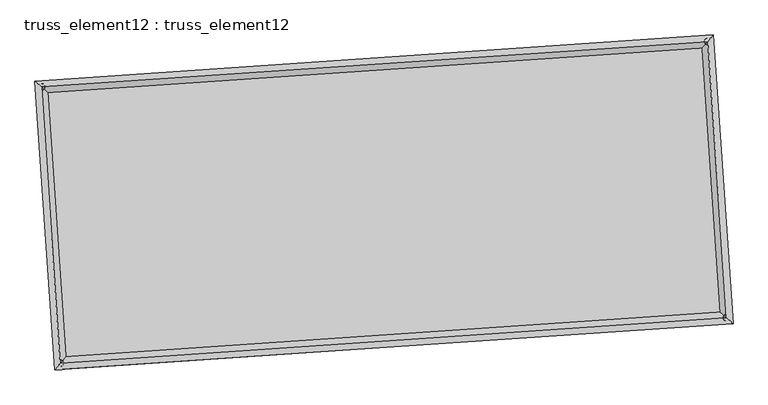
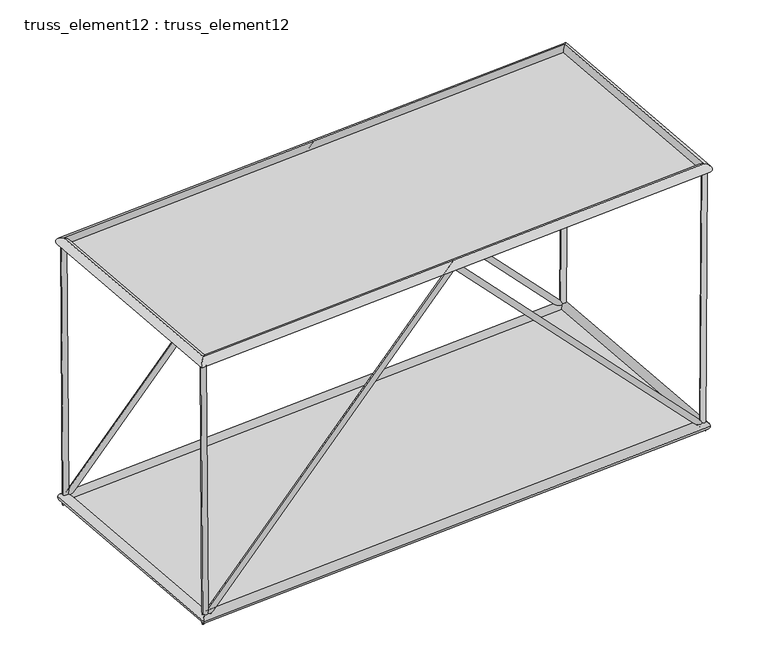
"""IFC4 building model written with IfcOpenShell, lengths in millimetres: plate geometry, truss_element12 : truss_element12."""

from ifc_helpers import new_model, si_unit, frame, origin, origin_with_axes, place, context, project, spatial, polyline, circle_curve, ellipse_curve, outline, extrude, source, transform, mapped, element, save
from ifc_brep_helpers import plane_surface, cylinder_surface, advanced_brep


def truss_element12_truss_element12_0bdd8d05(model_context):
    return source(origin(), model_context, "Body", "SolidModel", [
        advanced_brep(
        [(-3699.2780171, 2273.8827184, 5000.224961), (-3798.3790208, 2260.5216048, 4999.5381605), (-3665.7874801, 2276.1663109, 123.3255888), (-3763.1994027, 2262.9203692, -123.3255888), (1063.4543836, 2598.635336, 5072.0064394), (1063.9065449, 2592.0623743, 4927.760284), (5793.213407, 2921.1396243, 123.3293252), (5891.54757, 2921.2408642, -123.3293252), (5826.190706, 2923.388221, 5000.223301), (5926.1881888, 2923.6028763, 4999.5470243)],
        [
            (0, 1, circle_curve(frame((-3748.828519, 2267.2021616, 4999.8815607), z_axis=(-0.006867015509295821, -0.000468235683609246, 0.9999763121461127), x_axis=(-0.13361118718071577, 0.9910337254669442, -0.0004534834827120485)), 50.0)),
            (1, 0, circle_curve(frame((-3748.828519, 2267.2021616, 4999.8815607), z_axis=(-0.006867015509295821, -0.000468235683609246, 0.9999763121461127), x_axis=(-0.13361118718071577, 0.9910337254669442, -0.0004534834827120485)), 50.0)),
            (0, 2),
            (2, 3, ellipse_curve(frame((-3714.4934414, 2269.54334, 0.0), z_axis=(-0.927066716557074, -0.06321315529151074, 0.3695286187160306), x_axis=(0.3686725672674677, 0.025138380906336275, 0.9292193497500052)), 133.0085635, 50.0)),
            (3, 1),
            (3, 2, ellipse_curve(frame((-3714.4934414, 2269.54334, 0.0), z_axis=(-0.927066716557074, -0.06321315529151074, 0.3695286187160306), x_axis=(0.3686725672674677, 0.025138380906336275, 0.9292193497500052)), 133.0085635, 50.0)),
            (2, 4),
            (4, 5, ellipse_curve(frame((1063.6804642, 2595.3488551, 4999.8833617), z_axis=(-0.9976833956976204, -0.06802823820297604, -2.750026008393468e-05), x_axis=(2.7436552873218184e-05, 1.8707942446141108e-06, -0.9999999996218679)), 72.2801261, 50.0)),
            (5, 3),
            (5, 4, ellipse_curve(frame((1063.6804642, 2595.3488551, 4999.8833617), z_axis=(-0.9976833956976204, -0.06802823820297604, -2.750026008393468e-05), x_axis=(2.7436552873218184e-05, 1.8707942446141108e-06, -0.9999999996218679)), 72.2801261, 50.0)),
            (4, 6),
            (6, 7, ellipse_curve(frame((5842.3804885, 2921.1902443, 0.0), z_axis=(-0.9270371329382554, -0.06321113809700134, -0.3696031739231976), x_axis=(-0.368746949759749, -0.025143452765731062, 0.9291896974385255)), 133.0168379, 50.0)),
            (7, 5),
            (7, 6, ellipse_curve(frame((5842.3804885, 2921.1902443, 0.0), z_axis=(-0.9270371329382554, -0.06321113809700134, -0.3696031739231976), x_axis=(-0.368746949759749, -0.025143452765731062, 0.9291896974385255)), 133.0168379, 50.0)),
            (8, 9, circle_curve(frame((5876.1894474, 2923.4955486, 4999.8851627), z_axis=(0.006761791779643145, 0.0004610608774766411, 0.9999770325336459), x_axis=(-0.002149622020133885, 0.9999975898630503, -0.00044653472552298745)), 50.0)),
            (9, 8, circle_curve(frame((5876.1894474, 2923.4955486, 4999.8851627), z_axis=(0.006761791779643145, 0.0004610608774766411, 0.9999770325336459), x_axis=(-0.002149622020133885, 0.9999975898630503, -0.00044653472552298745)), 50.0)),
            (6, 8),
            (9, 7),
        ],
        [
            plane_surface(frame((-3748.828519, 2317.2021561, 4999.9049731), z_axis=(-0.006867015509297537, -0.0004682356836103226, 0.9999763121461126), x_axis=(0.9999764217710311, -3.215457516247967e-06, 0.006867014756483772))),
            cylinder_surface(frame((-3748.828519, 2267.2021616, 4999.8815607), z_axis=(-0.006867015509295821, -0.000468235683609246, 0.9999763121461127), x_axis=(-0.13361118718071577, 0.9910337254669442, -0.0004534834827120485)), 50.0),
            cylinder_surface(frame((-3714.4934414, 2269.54334, 0.0), z_axis=(-0.6901307509390465, -0.04705739247394388, -0.7221531336370847), x_axis=(-0.0204116303240351, 0.9987523729372, -0.04557480553800632)), 50.0),
            cylinder_surface(frame((1063.6804642, 2595.3488551, 4999.8833617), z_axis=(-0.6901703766804564, -0.04706009440261949, 0.7221150868577483), x_axis=(-0.11534672532663481, 0.9922791096910546, -0.04557742233990455)), 50.0),
            plane_surface(frame((5876.1894474, 2873.495554, 4999.9082162), z_axis=(0.006761791779644185, 0.00046106087747216243, 0.9999770325336457), x_axis=(0.9999771388246477, -3.1176689248013658e-06, -0.00676179106091013))),
            cylinder_surface(frame((5842.3804885, 2921.1902443, 0.0), z_axis=(-0.006761791779643143, -0.000461060877476641, -0.9999770325336457), x_axis=(-0.002149622020133885, 0.9999975898630503, -0.00044653472552298745)), 50.0),
        ],
        [
            (0, [[1, 2]]),
            (1, [[-1, 3, 4, 5]]),
            (1, [[-2, -5, 6, -3]]),
            (2, [[-4, 7, 8, 9]]),
            (2, [[-6, -9, 10, -7]]),
            (3, [[-8, 11, 12, 13]]),
            (3, [[-10, -13, 14, -11]]),
            (4, [[15, 16]]),
            (5, [[-12, 17, -16, 18]]),
            (5, [[-14, -18, -15, -17]]),
        ],
    ),
        advanced_brep(
        [(-3427.1650642, -1716.8508659, 5000.224961), (-3526.2660679, -1730.2119795, 4999.5381605), (-3393.6745272, -1714.5672734, 123.3255888), (-3491.0864498, -1727.8132151, -123.3255888), (1335.5673365, -1392.0982483, 5072.0064394), (1336.0194978, -1398.67121, 4927.760284), (6065.3263599, -1069.59396, 123.3293252), (6163.6605229, -1069.4927201, -123.3293252), (6098.3036589, -1067.3453633, 5000.223301), (6198.3011417, -1067.130708, 4999.5470243)],
        [
            (0, 1, circle_curve(frame((-3476.715566, -1723.5314227, 4999.8815607), z_axis=(-0.006867015509295706, -0.0004682356836092419, 0.9999763121461127), x_axis=(-0.13361118718071638, 0.9910337254669442, -0.0004534834827120414)), 50.0)),
            (1, 0, circle_curve(frame((-3476.715566, -1723.5314227, 4999.8815607), z_axis=(-0.006867015509295706, -0.0004682356836092419, 0.9999763121461127), x_axis=(-0.13361118718071638, 0.9910337254669442, -0.0004534834827120414)), 50.0)),
            (0, 2),
            (2, 3, ellipse_curve(frame((-3442.3804885, -1721.1902443, 0.0), z_axis=(-0.9270667165570737, -0.06321315529151104, 0.36952861871603054), x_axis=(0.36867256726746755, 0.02513838090633639, 0.9292193497500053)), 133.0085635, 50.0)),
            (3, 1),
            (3, 2, ellipse_curve(frame((-3442.3804885, -1721.1902443, 0.0), z_axis=(-0.9270667165570737, -0.06321315529151104, 0.36952861871603054), x_axis=(0.36867256726746755, 0.02513838090633639, 0.9292193497500053)), 133.0085635, 50.0)),
            (2, 4),
            (4, 5, ellipse_curve(frame((1335.7934171, -1395.3847292, 4999.8833617), z_axis=(-0.9976833956976204, -0.06802823820297628, -2.750026008401492e-05), x_axis=(2.743655287337192e-05, 1.8707942445372394e-06, -0.9999999996218679)), 72.2801261, 50.0)),
            (5, 3),
            (5, 4, ellipse_curve(frame((1335.7934171, -1395.3847292, 4999.8833617), z_axis=(-0.9976833956976204, -0.06802823820297628, -2.750026008401492e-05), x_axis=(2.743655287337192e-05, 1.8707942445372394e-06, -0.9999999996218679)), 72.2801261, 50.0)),
            (4, 6),
            (6, 7, ellipse_curve(frame((6114.4934414, -1069.54334, 0.0), z_axis=(-0.9270371329382552, -0.06321113809700153, -0.3696031739231974), x_axis=(-0.368746949759749, -0.025143452765731107, 0.9291896974385254)), 133.0168379, 50.0)),
            (7, 5),
            (7, 6, ellipse_curve(frame((6114.4934414, -1069.54334, 0.0), z_axis=(-0.9270371329382552, -0.06321113809700153, -0.3696031739231974), x_axis=(-0.368746949759749, -0.025143452765731107, 0.9291896974385254)), 133.0168379, 50.0)),
            (8, 9, circle_curve(frame((6148.3024003, -1067.2380357, 4999.8851627), z_axis=(0.006761791779642977, 0.0004610608774766668, 0.9999770325336459), x_axis=(-0.002149622020133642, 0.9999975898630503, -0.00044653472552301515)), 50.0)),
            (9, 8, circle_curve(frame((6148.3024003, -1067.2380357, 4999.8851627), z_axis=(0.006761791779642977, 0.0004610608774766668, 0.9999770325336459), x_axis=(-0.002149622020133642, 0.9999975898630503, -0.00044653472552301515)), 50.0)),
            (6, 8),
            (9, 7),
        ],
        [
            plane_surface(frame((-3476.715566, -1673.5314282, 4999.9049731), z_axis=(-0.006867015509297537, -0.0004682356836103226, 0.9999763121461126), x_axis=(0.9999764217710311, -3.215457516247967e-06, 0.006867014756483772))),
            cylinder_surface(frame((-3476.715566, -1723.5314227, 4999.8815607), z_axis=(-0.006867015509295706, -0.0004682356836092419, 0.9999763121461127), x_axis=(-0.13361118718071638, 0.9910337254669442, -0.0004534834827120414)), 50.0),
            cylinder_surface(frame((-3442.3804885, -1721.1902443, 0.0), z_axis=(-0.6901307509390463, -0.04705739247394409, -0.7221531336370847), x_axis=(-0.020411630324035174, 0.9987523729372, -0.04557480553800655)), 50.0),
            cylinder_surface(frame((1335.7934171, -1395.3847292, 4999.8833617), z_axis=(-0.6901703766804567, -0.04706009440261962, 0.7221150868577483), x_axis=(-0.1153467253266352, 0.9922791096910545, -0.04557742233990476)), 50.0),
            plane_surface(frame((6148.3024003, -1117.2380303, 4999.9082162), z_axis=(0.006761791779644185, 0.0004610608774721631, 0.9999770325336457), x_axis=(0.9999771388246477, -3.1176689248013658e-06, -0.00676179106091013))),
            cylinder_surface(frame((6114.4934414, -1069.54334, 0.0), z_axis=(-0.006761791779642976, -0.0004610608774766667, -0.9999770325336457), x_axis=(-0.002149622020133642, 0.9999975898630503, -0.00044653472552301515)), 50.0),
        ],
        [
            (0, [[1, 2]]),
            (1, [[-1, 3, 4, 5]]),
            (1, [[-2, -5, 6, -3]]),
            (2, [[-4, 7, 8, 9]]),
            (2, [[-6, -9, 10, -7]]),
            (3, [[-8, 11, 12, 13]]),
            (3, [[-10, -13, 14, -11]]),
            (4, [[15, 16]]),
            (5, [[-12, 17, -16, 18]]),
            (5, [[-14, -18, -15, -17]]),
        ],
    ),
        advanced_brep(
        [(-3476.7146152, -1723.5303688, 4909.8815607), (-3476.7165169, -1723.5324765, 5089.8815607), (-3748.8296041, 2267.2030767, 5089.8815607), (-3748.8274338, 2267.2012466, 4909.8815607), (5876.1903312, 2923.4965979, 5089.8851627), (5876.1885636, 2923.4944993, 4909.8851627), (6148.3034184, -1067.2389553, 5089.8851627), (6148.3013822, -1067.237116, 4909.8851627)],
        [
            (0, 1, ellipse_curve(frame((-3476.715566, -1723.5314227, 4999.8815607), z_axis=(-0.7535719234054068, 0.6573654662780862, -2.6400514555865953e-07), x_axis=(-0.6573654662780336, -0.7535719234054529, -2.640051451758168e-07)), 127.2792206, 90.0)),
            (1, 2),
            (2, 3, ellipse_curve(frame((-3748.828519, 2267.2021616, 4999.8815607), z_axis=(-0.6573654662780338, -0.7535719234054528, -2.6400514525519494e-07), x_axis=(0.7535719234054069, -0.6573654662780862, 2.640051456380377e-07)), 127.2792206, 90.0)),
            (3, 0),
            (1, 0, ellipse_curve(frame((-3476.715566, -1723.5314227, 4999.8815607), z_axis=(-0.7535719234054068, 0.6573654662780862, -2.6400514555865953e-07), x_axis=(-0.6573654662780336, -0.7535719234054529, -2.640051451758168e-07)), 127.2792206, 90.0)),
            (3, 2, ellipse_curve(frame((-3748.828519, 2267.2021616, 4999.8815607), z_axis=(-0.6573654662780338, -0.7535719234054528, -2.6400514525519494e-07), x_axis=(0.7535719234054069, -0.6573654662780862, 2.640051456380377e-07)), 127.2792206, 90.0)),
            (2, 4),
            (4, 5, ellipse_curve(frame((5876.1894474, 2923.4955486, 4999.8851627), z_axis=(-0.7535719234054068, 0.6573654662780863, -2.6400514544662063e-07), x_axis=(-0.6573654662780339, -0.7535719234054526, -2.6400514544661195e-07)), 127.2792206, 90.0)),
            (5, 3),
            (5, 4, ellipse_curve(frame((5876.1894474, 2923.4955486, 4999.8851627), z_axis=(-0.7535719234054068, 0.6573654662780863, -2.6400514544662063e-07), x_axis=(-0.6573654662780339, -0.7535719234054526, -2.6400514544661195e-07)), 127.2792206, 90.0)),
            (4, 6),
            (6, 7, ellipse_curve(frame((6148.3024003, -1067.2380357, 4999.8851627), z_axis=(0.6573654662780338, 0.7535719234054526, 2.6400514536723384e-07), x_axis=(-0.7535719234054067, 0.6573654662780865, -2.640051453672425e-07)), 127.2792206, 90.0)),
            (7, 5),
            (7, 6, ellipse_curve(frame((6148.3024003, -1067.2380357, 4999.8851627), z_axis=(0.6573654662780338, 0.7535719234054526, 2.6400514536723384e-07), x_axis=(-0.7535719234054067, 0.6573654662780865, -2.640051453672425e-07)), 127.2792206, 90.0)),
            (6, 1),
            (0, 7),
        ],
        [
            cylinder_surface(frame((-3476.715566, -1723.5314227, 4999.8815607), z_axis=(0.0680282382286978, -0.9976833960748769, 0.0), x_axis=(-0.9976833960107591, -0.06802823822432585, -1.1337253580804916e-05)), 90.0),
            cylinder_surface(frame((-3748.828519, 2267.2021616, 4999.8815607), z_axis=(-0.9976833960748073, -0.06802823822869414, -3.7335965722688633e-07), x_axis=(-0.06802823822052616, 0.997683396015191, -1.0963893923871191e-05)), 90.0),
            cylinder_surface(frame((5876.1894474, 2923.4955486, 4999.8851627), z_axis=(-0.06802823822869772, 0.9976833960748769, 0.0), x_axis=(0.9976833960189271, 0.06802823822488271, -1.0590534266666754e-05)), 90.0),
            cylinder_surface(frame((6148.3024003, -1067.2380357, 4999.8851627), z_axis=(0.9976833960748072, 0.06802823822869412, 3.733596571146287e-07), x_axis=(0.06802823822869412, -0.997683396014634, -1.0963893923758946e-05)), 90.0),
        ],
        [
            (0, [[1, 2, 3, 4]]),
            (0, [[5, -4, 6, -2]]),
            (1, [[-3, 7, 8, 9]]),
            (1, [[-6, -9, 10, -7]]),
            (2, [[-8, 11, 12, 13]]),
            (2, [[-10, -13, 14, -11]]),
            (3, [[-12, 15, -1, 16]]),
            (3, [[-14, -16, -5, -15]]),
        ],
    ),
        advanced_brep(
        [(-3358.7115243, -1625.2761972, 0.0), (-3526.0494527, -1817.1042913, 0.0), (-3810.4074885, 2353.2123043, 0.0), (-3618.5793943, 2185.8743758, 0.0), (5926.0494527, 3017.1042913, 0.0), (5758.7115243, 2825.2761972, 0.0), (6210.4074885, -1153.2123043, 0.0), (6018.5793943, -985.8743758, 0.0)],
        [
            (0, 1, ellipse_curve(frame((-3442.3804885, -1721.1902443, 0.0), z_axis=(-0.7535719234054564, 0.6573654662780825, 0.0), x_axis=(-0.6573654662780822, -0.7535719234054566, 0.0)), 127.2792206, 90.0)),
            (1, 2),
            (2, 3, ellipse_curve(frame((-3714.4934414, 2269.54334, 0.0), z_axis=(-0.6573654662780825, -0.7535719234054565, 0.0), x_axis=(0.7535719234054564, -0.6573654662780825, 0.0)), 127.2792206, 90.0)),
            (3, 0),
            (1, 0, ellipse_curve(frame((-3442.3804885, -1721.1902443, 0.0), z_axis=(-0.7535719234054564, 0.6573654662780825, 0.0), x_axis=(-0.6573654662780822, -0.7535719234054566, 0.0)), 127.2792206, 90.0)),
            (3, 2, ellipse_curve(frame((-3714.4934414, 2269.54334, 0.0), z_axis=(-0.6573654662780825, -0.7535719234054565, 0.0), x_axis=(0.7535719234054564, -0.6573654662780825, 0.0)), 127.2792206, 90.0)),
            (2, 4),
            (4, 5, ellipse_curve(frame((5842.3804885, 2921.1902443, 0.0), z_axis=(-0.7535719234054564, 0.6573654662780825, 0.0), x_axis=(-0.6573654662780826, -0.7535719234054563, 0.0)), 127.2792206, 90.0)),
            (5, 3),
            (5, 4, ellipse_curve(frame((5842.3804885, 2921.1902443, 0.0), z_axis=(-0.7535719234054564, 0.6573654662780825, 0.0), x_axis=(-0.6573654662780826, -0.7535719234054563, 0.0)), 127.2792206, 90.0)),
            (4, 6),
            (6, 7, ellipse_curve(frame((6114.4934414, -1069.54334, 0.0), z_axis=(0.6573654662780827, 0.7535719234054565, 0.0), x_axis=(-0.7535719234054566, 0.6573654662780823, 0.0)), 127.2792206, 90.0)),
            (7, 5),
            (7, 6, ellipse_curve(frame((6114.4934414, -1069.54334, 0.0), z_axis=(0.6573654662780827, 0.7535719234054565, 0.0), x_axis=(-0.7535719234054566, 0.6573654662780823, 0.0)), 127.2792206, 90.0)),
            (6, 1),
            (0, 7),
        ],
        [
            cylinder_surface(frame((-3442.3804885, -1721.1902443, 0.0), z_axis=(0.0680282382286986, -0.9976833960748768, 0.0), x_axis=(-0.9976833960748768, -0.0680282382286986, 0.0)), 90.0),
            cylinder_surface(frame((-3714.4934414, 2269.54334, 0.0), z_axis=(-0.9976833960748768, -0.06802823822869966, 0.0), x_axis=(-0.06802823822869966, 0.9976833960748768, 0.0)), 90.0),
            cylinder_surface(frame((5842.3804885, 2921.1902443, 0.0), z_axis=(-0.06802823822869838, 0.9976833960748769, 0.0), x_axis=(0.9976833960748769, 0.06802823822869838, 0.0)), 90.0),
            cylinder_surface(frame((6114.4934414, -1069.54334, 0.0), z_axis=(0.9976833960748768, 0.06802823822869936, 0.0), x_axis=(0.06802823822869936, -0.9976833960748768, 0.0)), 90.0),
        ],
        [
            (0, [[1, 2, 3, 4]]),
            (0, [[5, -4, 6, -2]]),
            (1, [[-3, 7, 8, 9]]),
            (1, [[-6, -9, 10, -7]]),
            (2, [[-8, 11, 12, 13]]),
            (2, [[-10, -13, 14, -11]]),
            (3, [[-12, 15, -1, 16]]),
            (3, [[-14, -16, -5, -15]]),
        ],
    ),
        extrude(outline(polyline([(-3442.3804885, -1721.1902443), (-3714.4934414, 2269.54334), (5842.3804885, 2921.1902443), (6114.4934414, -1069.54334), (-3442.3804885, -1721.1902443)])), origin_with_axes(), (0.0, 0.0, 1.0), 20.0),
        extrude(outline(polyline([(-2000.0, 4823.6835474), (2000.0, 4823.6835475), (1999.9999999, -4823.6835474), (-2000.0000001, -4823.6835474), (-2000.0, 4823.6835474)])), frame((1199.7369407, 599.982063, 4999.8833617), z_axis=(-3.72494730797882e-07, -2.539899943672577e-08, 0.9999999999999304), x_axis=(-0.06802823822869852, 0.9976833960748768, 0.0)), (0.0, 0.0, 1.0), 20.0),
    ])


if __name__ == "__main__":
    model = new_model("IFC4")
    model_context = context("Model", 3, world=origin())
    ifc_project = project(units=[si_unit("LENGTHUNIT", "METRE", prefix="MILLI")], contexts=[model_context])
    site = spatial("IfcSite", under=ifc_project)
    building = spatial("IfcBuilding", under=site)
    placement = place(None, origin())
    truss_element12_truss_element12_shape = truss_element12_truss_element12_0bdd8d05(model_context)
    element("IfcPlate", 1, ObjectType="truss_element12 : truss_element12", at=placement, inside=building, context=model_context, shape_type="MappedRepresentation", body=[
        mapped(truss_element12_truss_element12_shape, transform((0.0, 0.0, 0.0), x_axis=(1.0, 0.0, 0.0), y_axis=(0.0, 1.0, 0.0), z_axis=(0.0, 0.0, 1.0))),
    ])
    save(model, "model.ifc")

# Revit data of these elements
# Type "truss_element12 : truss_element12"
#   steellbar1 = 90 mm
#   steelbar2 = 50 mm
#   offset1 = 5000 mm
#   M = Default Roof
# Element 1 (IfcPlate, "truss_element12 : truss_element12")
#   Materials on its faces: "Default Roof"
# Materials
#   "Default Roof": class "Miscellaneous", colour RGB 0 127 0, transparency 0, Comments = "Rendering appearance not upgraded Rendering appearance not upgraded ", Cost = 0
